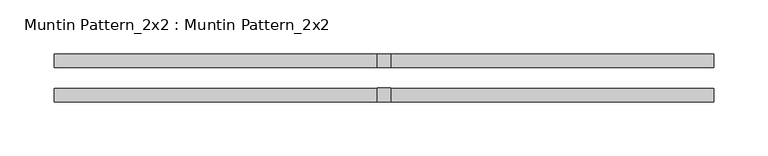
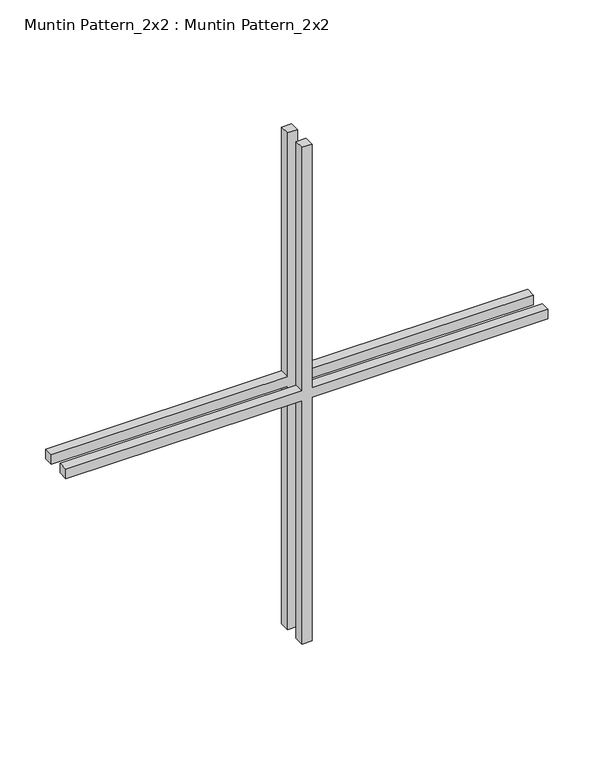
"""IFC4 building model written with IfcOpenShell, lengths in millimetres: proxy geometry, Muntin Pattern_2x2 : Muntin Pattern_2x2."""

from ifc_helpers import new_model, si_unit, frame, origin, place, context, project, spatial, polyline, outline, extrude, source, transform, mapped, element, save


def muntin_pattern_2x2_muntin_pattern_2x2_550b37bf(model_context):
    return source(origin(), model_context, "Body", "SweptSolid", [
        extrude(outline(polyline([(338.1375, -6.35), (338.1375, -304.8), (325.4375, -304.8), (325.4375, -6.35), (0.0, -6.35), (0.0, 6.35), (325.4375, 6.35), (325.4375, 304.8), (338.1375, 304.8), (338.1375, 6.35), (663.575, 6.35), (663.575, -6.35), (338.1375, -6.35)])), frame((0.0, 9.525, 0.0), z_axis=(0.0, 1.0, 0.0), x_axis=(0.0, 0.0, 1.0)), (0.0, 0.0, 1.0), 12.7),
        extrude(outline(polyline([(338.1375, -6.35), (338.1375, -304.8), (325.4375, -304.8), (325.4375, -6.35), (0.0, -6.35), (0.0, 6.35), (325.4375, 6.35), (325.4375, 304.8), (338.1375, 304.8), (338.1375, 6.35), (663.575, 6.35), (663.575, -6.35), (338.1375, -6.35)])), frame((0.0, -22.225, 0.0), z_axis=(0.0, 1.0, 0.0), x_axis=(0.0, 0.0, 1.0)), (0.0, 0.0, 1.0), 12.7),
    ])


if __name__ == "__main__":
    model = new_model("IFC4")
    model_context = context("Model", 3, world=origin())
    ifc_project = project(units=[si_unit("LENGTHUNIT", "METRE", prefix="MILLI")], contexts=[model_context])
    site = spatial("IfcSite", under=ifc_project)
    building = spatial("IfcBuilding", under=site)
    placement = place(None, origin())
    muntin_pattern_2x2_muntin_pattern_2x2_shape = muntin_pattern_2x2_muntin_pattern_2x2_550b37bf(model_context)
    element("IfcBuildingElementProxy", 1, Name="Muntin Pattern_2x2 : Muntin Pattern_2x2", ObjectType="Muntin Pattern_2x2 : Muntin Pattern_2x2", at=placement, inside=building, context=model_context, shape_type="MappedRepresentation", body=[
        mapped(muntin_pattern_2x2_muntin_pattern_2x2_shape, transform((0.0, 0.0, 0.0), x_axis=(1.0, 0.0, 0.0), y_axis=(0.0, 1.0, 0.0), z_axis=(0.0, 0.0, 1.0))),
    ])
    save(model, "model.ifc")

# Revit data of these elements
# Type "Muntin Pattern_2x2 : Muntin Pattern_2x2"
#   Width [instance default] = 4' - 0"
#   Thickness = 0' - 0 1/2"
#   Height [instance default] = 4' - 0"
#   Distance = 0' - 0 3/4"
#   Interior Material [instance default] = none
#   Exterior Material [instance default] = none
#   Default Elevation = 0
# Element 1 (IfcBuildingElementProxy, "Muntin Pattern_2x2 : Muntin Pattern_2x2")
#   Width = 2' - 0"
#   Height = 2' - 2 1/8"
#   Interior Material = Wood - Stained
#   Exterior Material = Clad - White
#   Materials on its faces: "Clad - White", "Wood - Stained"
# Materials
#   "Clad - White": class "Wood", colour RGB 242 242 238, transparency 0, Cost = 0
#   "Wood - Stained": class "Wood", colour RGB 224 178 126, transparency 0, Cost = 0
